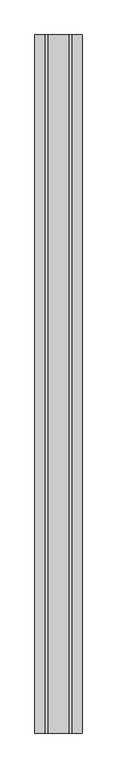
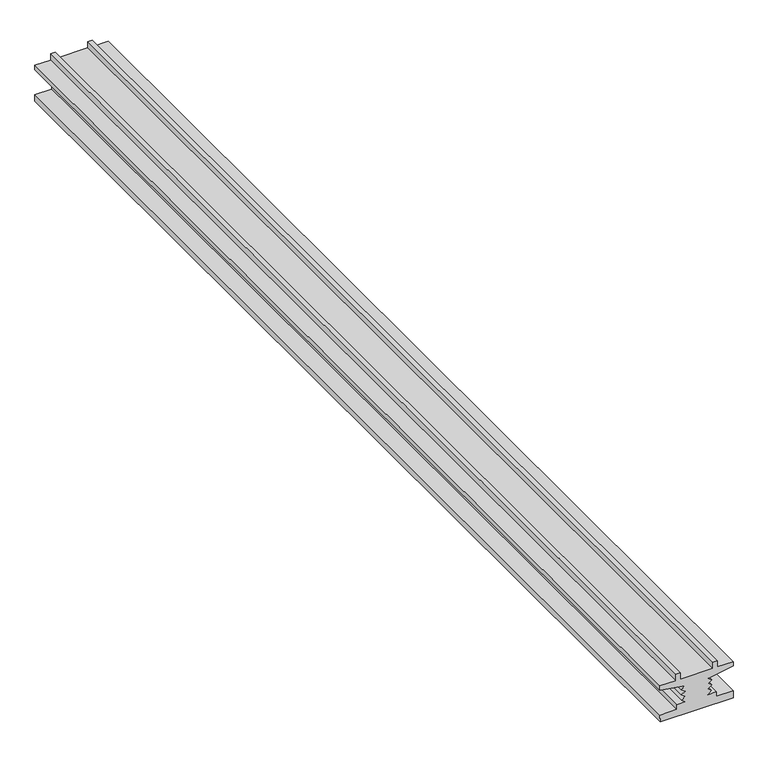
"""IFC4 building model written with IfcOpenShell, lengths in millimetres: proxy geometry, Bison pedestal : Bison pedestal."""

from ifc_helpers import new_model, si_unit, frame, origin, place, context, project, spatial, polyline, outline, extrude, source, transform, mapped, element, save


def generic_models_200ae2cb(model_context):
    return source(origin(), model_context, "Body", "SweptSolid", [
        extrude(outline(polyline([(36442.3966729, -5430.850316), (36455.796875, -5430.7211914), (36455.796875, -5461.5600586), (36464.75225, -5461.5600586), (36464.75225, -5477.7421875), (36470.6350625, -5470.6806641), (36475.7874062, -5477.3007812), (36481.2288125, -5470.2397461), (36486.37725, -5477.0068359), (36491.4436562, -5469.8574219), (36496.5374062, -5476.2905273), (36504.3108437, -5430.7211914), (36512.6194375, -5430.7211914), (36512.6194375, -5460.2075195), (36524.9514687, -5460.2075195), (36524.9514687, -5467.980957), (36512.6194375, -5467.980957), (36512.6194375, -5528.5610352), (36524.9514687, -5528.5610352), (36524.9514687, -5536.3344727), (36512.6194375, -5536.3344727), (36512.6194375, -5565.8208008), (36504.3108437, -5565.8208008), (36496.5374062, -5520.2514648), (36491.4436562, -5526.6845703), (36486.37725, -5519.5351562), (36481.2288125, -5526.3022461), (36475.7874062, -5519.2412109), (36470.6350625, -5525.8613281), (36464.75225, -5518.7998047), (36464.75225, -5534.9819336), (36455.796875, -5534.9819336), (36455.796875, -5565.8208008), (36442.3966729, -5565.6916762), (36442.3966729, -5498.2709961), (36442.3966729, -5430.850316)])), frame((0.0, -1052.8906574, 0.0), z_axis=(0.0, 1.0, 0.0), x_axis=(0.0, 0.0, 1.0)), (0.0, 0.0, 1.0), 2000.0),
    ])


if __name__ == "__main__":
    model = new_model("IFC4")
    model_context = context("Model", 3, world=origin())
    ifc_project = project(units=[si_unit("LENGTHUNIT", "METRE", prefix="MILLI")], contexts=[model_context])
    site = spatial("IfcSite", under=ifc_project)
    building = spatial("IfcBuilding", under=site)
    placement = place(None, origin())
    generic_models_shape = generic_models_200ae2cb(model_context)
    element("IfcBuildingElementProxy", 1, Name="Bison pedestal : Bison pedestal", ObjectType="Bison pedestal : Bison pedestal", at=placement, inside=building, context=model_context, shape_type="MappedRepresentation", body=[
        mapped(generic_models_shape, transform((0.0, 0.0, 0.0), x_axis=(1.0, 0.0, 0.0), y_axis=(0.0, 1.0, 0.0), z_axis=(0.0, 0.0, 1.0))),
    ])
    save(model, "model.ifc")

# Revit data of these elements
# Type "Bison pedestal : Bison pedestal"
#   NameOverride = "Bison pedestal"
# Element 1 (IfcBuildingElementProxy, "Bison pedestal : Bison pedestal")
#   Materials on its faces: "BUZON PEDESTAL"
# Materials
#   "BUZON PEDESTAL": class "Unassigned", colour RGB 66 66 66, transparency 0
